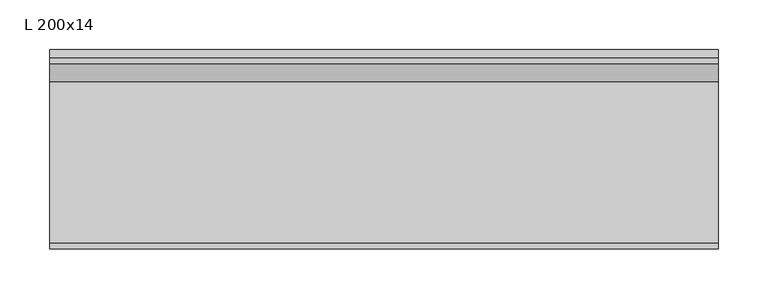
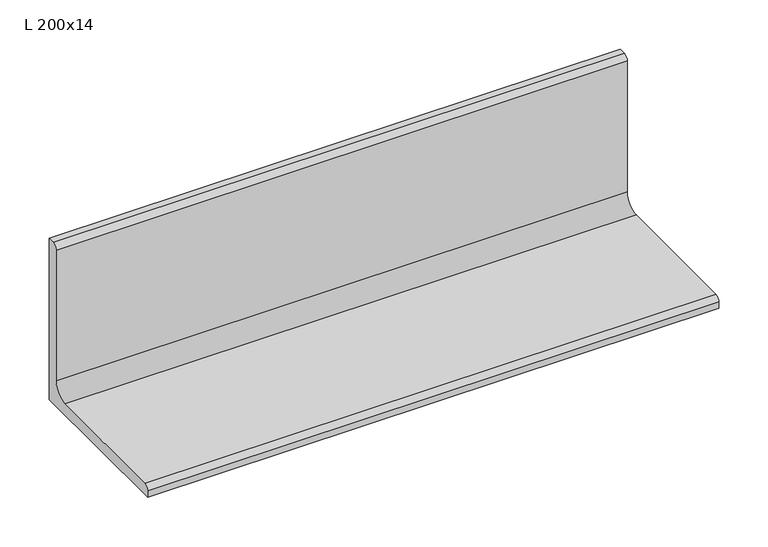
"""IFC4 building model written with IfcOpenShell, lengths in millimetres: beam geometry, Уголок (ГОСТ 8509-93) Балки : L 200x14."""

from ifc_helpers import new_model, si_unit, point, frame, frame_2d, origin, place, context, project, spatial, polyline, circle_curve, trimmed, segment, composite_curve, outline, extrude, source, transform, mapped, element, save


def l_200x14_1023fe27(model_context):
    return source(origin(), model_context, "Body", "SweptSolid", [
        extrude(outline(composite_curve([segment(polyline([(54.6, -54.6), (-145.4, -54.6), (-145.4, -46.6)]), True, "CONTINUOUS"), segment(trimmed(circle_curve(frame_2d((-139.4, -46.6)), 6.0), [point((-145.4, -46.6))], [point((-139.4, -40.6))], False, "CARTESIAN"), True, "CONTINUOUS"), segment(polyline([(-139.4, -40.6), (22.6, -40.6)]), True, "CONTINUOUS"), segment(trimmed(circle_curve(frame_2d((22.6, -22.6)), 18.0), [point((22.6, -40.6))], [point((40.6, -22.6))], True, "CARTESIAN"), True, "CONTINUOUS"), segment(polyline([(40.6, -22.6), (40.6, 139.4)]), True, "CONTINUOUS"), segment(trimmed(circle_curve(frame_2d((46.6, 139.4)), 6.0), [point((40.6, 139.4))], [point((46.6, 145.4))], False, "CARTESIAN"), True, "CONTINUOUS"), segment(polyline([(46.6, 145.4), (54.6, 145.4), (54.6, -54.6)]), True, "CONTINUOUS")], self_intersect=False)), frame((-335.0, 0.0, 0.0), z_axis=(1.0, 0.0, 0.0), x_axis=(0.0, 1.0, 0.0)), (0.0, 0.0, 1.0), 670.0),
    ])


if __name__ == "__main__":
    model = new_model("IFC4")
    model_context = context("Model", 3, world=origin())
    ifc_project = project(units=[si_unit("LENGTHUNIT", "METRE", prefix="MILLI")], contexts=[model_context])
    site = spatial("IfcSite", under=ifc_project)
    building = spatial("IfcBuilding", under=site)
    placement = place(None, origin())
    l_200x14_shape = l_200x14_1023fe27(model_context)
    element("IfcBeam", 1, ObjectType="Уголок (ГОСТ 8509-93) Балки : L 200x14", at=placement, inside=building, context=model_context, shape_type="MappedRepresentation", body=[
        mapped(l_200x14_shape, transform((0.0, 0.0, 0.0), x_axis=(1.0, 0.0, 0.0), y_axis=(0.0, 1.0, 0.0), z_axis=(0.0, 0.0, 1.0))),
    ])
    save(model, "model.ifc")

# Revit data of these elements
# Type "Уголок (ГОСТ 8509-93) Балки : L 200x14"
#   ri = 6 mm
#   ra = 18 mm
#   W = 0.419725
#   Vz = 145.4 mm
#   Vy = 145.4 mm
#   Vpz = 54.6 mm
#   Vpy = 54.6 mm
#   Length [instance default] = 1500 mm
#   bf = 200 mm
#   d = 200 mm
#   tf = 14 mm
#   tw = 14 mm
#   A = 0.00546 m²
#   Structural Material [instance default] = Металл - Сталь - 345 МПa
#   Assembly Code = ""
# Element 1 (IfcBeam, "Уголок (ГОСТ 8509-93) Балки : L 200x14")
#   Structural Material = C235
#   Materials on its faces: "C235"
# Materials
#   "Металл - Сталь - 345 МПa": class "Металл", colour RGB 247 247 247, transparency 0
#   "C235": class "Не назначено", colour RGB 0 0 0, transparency 0
